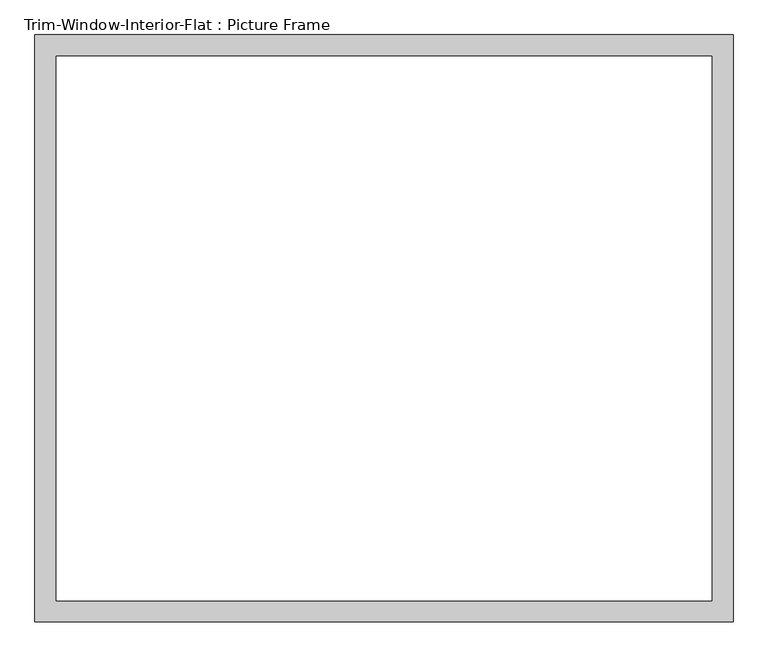
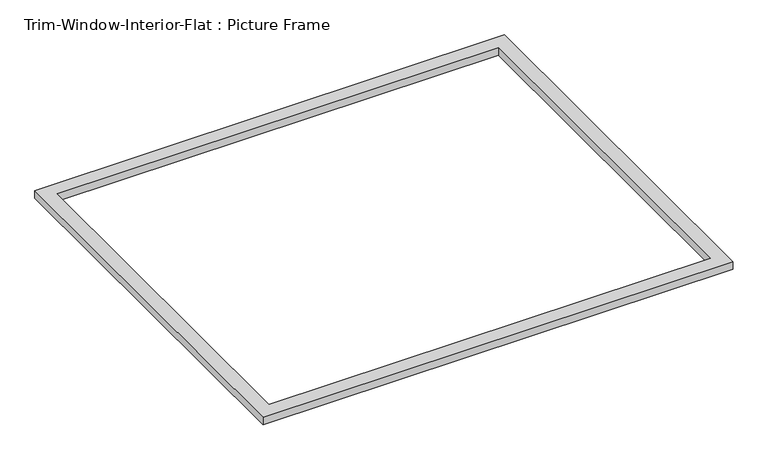
"""IFC4 building model written with IfcOpenShell, lengths in millimetres: proxy geometry, Trim-Window-Interior-Flat : Picture Frame."""

from ifc_helpers import new_model, si_unit, origin, origin_with_axes, place, context, project, spatial, polyline, outline, extrude, source, transform, mapped, element, save


def trim_window_interior_flat_picture_frame_f7c799ac(model_context):
    return source(origin(), model_context, "Body", "SweptSolid", [
        extrude(outline(polyline([(944.45, 44.45), (944.45, -1544.45), (-944.45, -1544.45), (-944.45, 44.45), (944.45, 44.45)]), holes=[polyline([(887.3, -12.7), (-887.3, -12.7), (-887.3, -1487.3), (887.3, -1487.3), (887.3, -12.7)])]), origin_with_axes(), (0.0, 0.0, 1.0), 31.75),
    ])


if __name__ == "__main__":
    model = new_model("IFC4")
    model_context = context("Model", 3, world=origin())
    ifc_project = project(units=[si_unit("LENGTHUNIT", "METRE", prefix="MILLI")], contexts=[model_context])
    site = spatial("IfcSite", under=ifc_project)
    building = spatial("IfcBuilding", under=site)
    placement = place(None, origin())
    trim_window_interior_flat_picture_frame_shape = trim_window_interior_flat_picture_frame_f7c799ac(model_context)
    element("IfcBuildingElementProxy", 1, Name="Trim-Window-Interior-Flat : Picture Frame", ObjectType="Trim-Window-Interior-Flat : Picture Frame", at=placement, inside=building, context=model_context, shape_type="MappedRepresentation", body=[
        mapped(trim_window_interior_flat_picture_frame_shape, transform((0.0, 0.0, 0.0), x_axis=(1.0, 0.0, 0.0), y_axis=(0.0, 1.0, 0.0), z_axis=(0.0, 0.0, 1.0))),
    ])
    save(model, "model.ifc")

# Revit data of these elements
# Type "Trim-Window-Interior-Flat : Picture Frame"
#   Trim Thickness_Picture Frame = 3.175 cm
#   Trim Width = 5.715 cm
#   Trim Thickness_with Sill = 1.905 cm
#   Sill Thickness = 3.175 cm
#   Opening Width [instance default] = 60.96 cm
#   Opening Height [instance default] = 91.44 cm
#   Default Elevation = 121.92 cm
#   Sill = no
#   Picture Frame = yes
#   Trim Material [instance default] = none
# Element 1 (IfcBuildingElementProxy, "Trim-Window-Interior-Flat : Picture Frame")
#   Opening Width = 180 cm
#   Opening Height = 150 cm
#   Trim Material = Wood - Stained
#   Materials on its faces: "Wood - Stained"
# Materials
#   "Wood - Stained": class "Wood", colour RGB 224 178 126, transparency 0, Cost = 0
